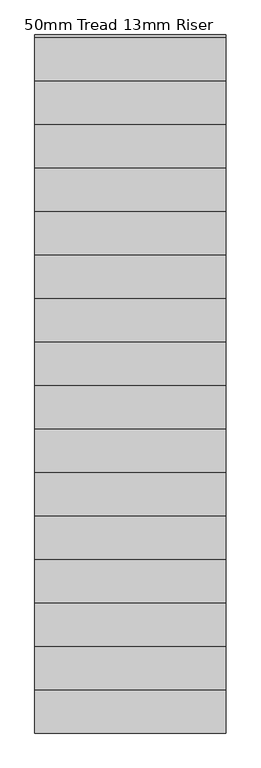
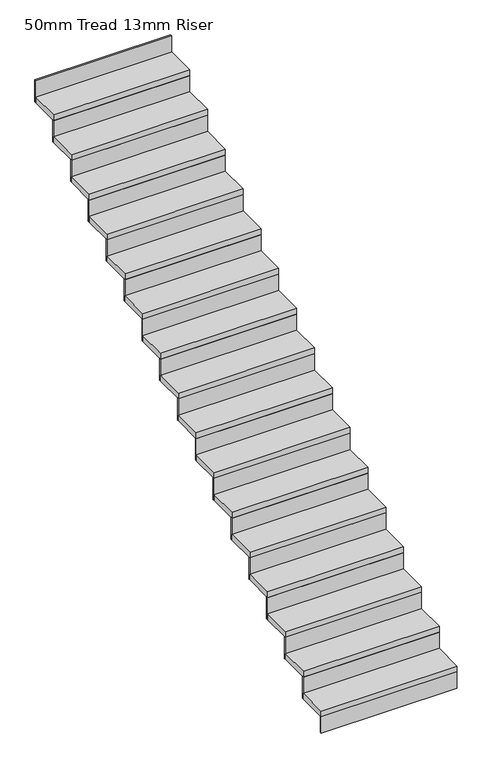
"""IFC4 building model written with IfcOpenShell, lengths in millimetres: stair flight geometry, 50mm Tread 13mm Riser."""

from ifc_helpers import new_model, si_unit, frame, origin, origin_with_axes, place, context, project, spatial, polyline, outline, extrude, source, transform, mapped, element, save


def stair_flight_50mm_tread_13mm_riser_fc77365a(model_context):
    return source(origin(), model_context, "Body", "SweptSolid", [
        extrude(outline(polyline([(-1832.0143079, -7091.702269), (-1832.0143079, -7104.202269), (-2932.0143079, -7104.202269), (-2932.0143079, -7091.702269), (-1832.0143079, -7091.702269)])), origin_with_axes(), (0.0, 0.0, 1.0), 138.2352941),
        extrude(outline(polyline([(-2932.0143079, -6854.202269), (-1832.0143079, -6854.202269), (-1832.0143079, -7104.202269), (-2932.0143079, -7104.202269), (-2932.0143079, -6854.202269)])), frame((0.0, 0.0, 138.2352941), z_axis=(0.0, 0.0, 1.0), x_axis=(1.0, 0.0, 0.0)), (0.0, 0.0, 1.0), 50.0),
        extrude(outline(polyline([(-1832.0143079, -6841.702269), (-1832.0143079, -6854.202269), (-2932.0143079, -6854.202269), (-2932.0143079, -6841.702269), (-1832.0143079, -6841.702269)])), frame((0.0, 0.0, 138.2352941), z_axis=(0.0, 0.0, 1.0), x_axis=(1.0, 0.0, 0.0)), (0.0, 0.0, 1.0), 188.2352941),
        extrude(outline(polyline([(-2932.0143079, -6604.202269), (-1832.0143079, -6604.202269), (-1832.0143079, -6854.202269), (-2932.0143079, -6854.202269), (-2932.0143079, -6604.202269)])), frame((0.0, 0.0, 326.4705882), z_axis=(0.0, 0.0, 1.0), x_axis=(1.0, 0.0, 0.0)), (0.0, 0.0, 1.0), 50.0),
        extrude(outline(polyline([(-1832.0143079, -6591.702269), (-1832.0143079, -6604.202269), (-2932.0143079, -6604.202269), (-2932.0143079, -6591.702269), (-1832.0143079, -6591.702269)])), frame((0.0, 0.0, 326.4705882), z_axis=(0.0, 0.0, 1.0), x_axis=(1.0, 0.0, 0.0)), (0.0, 0.0, 1.0), 188.2352941),
        extrude(outline(polyline([(-2932.0143079, -6354.202269), (-1832.0143079, -6354.202269), (-1832.0143079, -6604.202269), (-2932.0143079, -6604.202269), (-2932.0143079, -6354.202269)])), frame((0.0, 0.0, 514.7058824), z_axis=(0.0, 0.0, 1.0), x_axis=(1.0, 0.0, 0.0)), (0.0, 0.0, 1.0), 50.0),
        extrude(outline(polyline([(-1832.0143079, -6341.702269), (-1832.0143079, -6354.202269), (-2932.0143079, -6354.202269), (-2932.0143079, -6341.702269), (-1832.0143079, -6341.702269)])), frame((0.0, 0.0, 514.7058824), z_axis=(0.0, 0.0, 1.0), x_axis=(1.0, 0.0, 0.0)), (0.0, 0.0, 1.0), 188.2352941),
        extrude(outline(polyline([(-2932.0143079, -6104.202269), (-1832.0143079, -6104.202269), (-1832.0143079, -6354.202269), (-2932.0143079, -6354.202269), (-2932.0143079, -6104.202269)])), frame((0.0, 0.0, 702.9411765), z_axis=(0.0, 0.0, 1.0), x_axis=(1.0, 0.0, 0.0)), (0.0, 0.0, 1.0), 50.0),
        extrude(outline(polyline([(-1832.0143079, -6091.702269), (-1832.0143079, -6104.202269), (-2932.0143079, -6104.202269), (-2932.0143079, -6091.702269), (-1832.0143079, -6091.702269)])), frame((0.0, 0.0, 702.9411765), z_axis=(0.0, 0.0, 1.0), x_axis=(1.0, 0.0, 0.0)), (0.0, 0.0, 1.0), 188.2352941),
        extrude(outline(polyline([(-2932.0143079, -5854.202269), (-1832.0143079, -5854.202269), (-1832.0143079, -6104.202269), (-2932.0143079, -6104.202269), (-2932.0143079, -5854.202269)])), frame((0.0, 0.0, 891.1764706), z_axis=(0.0, 0.0, 1.0), x_axis=(1.0, 0.0, 0.0)), (0.0, 0.0, 1.0), 50.0),
        extrude(outline(polyline([(-1832.0143079, -5841.702269), (-1832.0143079, -5854.202269), (-2932.0143079, -5854.202269), (-2932.0143079, -5841.702269), (-1832.0143079, -5841.702269)])), frame((0.0, 0.0, 891.1764706), z_axis=(0.0, 0.0, 1.0), x_axis=(1.0, 0.0, 0.0)), (0.0, 0.0, 1.0), 188.2352941),
        extrude(outline(polyline([(-2932.0143079, -5604.202269), (-1832.0143079, -5604.202269), (-1832.0143079, -5854.202269), (-2932.0143079, -5854.202269), (-2932.0143079, -5604.202269)])), frame((0.0, 0.0, 1079.4117647), z_axis=(0.0, 0.0, 1.0), x_axis=(1.0, 0.0, 0.0)), (0.0, 0.0, 1.0), 50.0),
        extrude(outline(polyline([(-1832.0143079, -5591.702269), (-1832.0143079, -5604.202269), (-2932.0143079, -5604.202269), (-2932.0143079, -5591.702269), (-1832.0143079, -5591.702269)])), frame((0.0, 0.0, 1079.4117647), z_axis=(0.0, 0.0, 1.0), x_axis=(1.0, 0.0, 0.0)), (0.0, 0.0, 1.0), 188.2352941),
        extrude(outline(polyline([(-2932.0143079, -5354.202269), (-1832.0143079, -5354.202269), (-1832.0143079, -5604.202269), (-2932.0143079, -5604.202269), (-2932.0143079, -5354.202269)])), frame((0.0, 0.0, 1267.6470588), z_axis=(0.0, 0.0, 1.0), x_axis=(1.0, 0.0, 0.0)), (0.0, 0.0, 1.0), 50.0),
        extrude(outline(polyline([(-1832.0143079, -5341.702269), (-1832.0143079, -5354.202269), (-2932.0143079, -5354.202269), (-2932.0143079, -5341.702269), (-1832.0143079, -5341.702269)])), frame((0.0, 0.0, 1267.6470588), z_axis=(0.0, 0.0, 1.0), x_axis=(1.0, 0.0, 0.0)), (0.0, 0.0, 1.0), 188.2352941),
        extrude(outline(polyline([(-2932.0143079, -5104.202269), (-1832.0143079, -5104.202269), (-1832.0143079, -5354.202269), (-2932.0143079, -5354.202269), (-2932.0143079, -5104.202269)])), frame((0.0, 0.0, 1455.8823529), z_axis=(0.0, 0.0, 1.0), x_axis=(1.0, 0.0, 0.0)), (0.0, 0.0, 1.0), 50.0),
        extrude(outline(polyline([(-1832.0143079, -5091.702269), (-1832.0143079, -5104.202269), (-2932.0143079, -5104.202269), (-2932.0143079, -5091.702269), (-1832.0143079, -5091.702269)])), frame((0.0, 0.0, 1455.8823529), z_axis=(0.0, 0.0, 1.0), x_axis=(1.0, 0.0, 0.0)), (0.0, 0.0, 1.0), 188.2352941),
        extrude(outline(polyline([(-2932.0143079, -4854.202269), (-1832.0143079, -4854.202269), (-1832.0143079, -5104.202269), (-2932.0143079, -5104.202269), (-2932.0143079, -4854.202269)])), frame((0.0, 0.0, 1644.1176471), z_axis=(0.0, 0.0, 1.0), x_axis=(1.0, 0.0, 0.0)), (0.0, 0.0, 1.0), 50.0),
        extrude(outline(polyline([(-1832.0143079, -4841.702269), (-1832.0143079, -4854.202269), (-2932.0143079, -4854.202269), (-2932.0143079, -4841.702269), (-1832.0143079, -4841.702269)])), frame((0.0, 0.0, 1644.1176471), z_axis=(0.0, 0.0, 1.0), x_axis=(1.0, 0.0, 0.0)), (0.0, 0.0, 1.0), 188.2352941),
        extrude(outline(polyline([(-2932.0143079, -4604.202269), (-1832.0143079, -4604.202269), (-1832.0143079, -4854.202269), (-2932.0143079, -4854.202269), (-2932.0143079, -4604.202269)])), frame((0.0, 0.0, 1832.3529412), z_axis=(0.0, 0.0, 1.0), x_axis=(1.0, 0.0, 0.0)), (0.0, 0.0, 1.0), 50.0),
        extrude(outline(polyline([(-1832.0143079, -4591.702269), (-1832.0143079, -4604.202269), (-2932.0143079, -4604.202269), (-2932.0143079, -4591.702269), (-1832.0143079, -4591.702269)])), frame((0.0, 0.0, 1832.3529412), z_axis=(0.0, 0.0, 1.0), x_axis=(1.0, 0.0, 0.0)), (0.0, 0.0, 1.0), 188.2352941),
        extrude(outline(polyline([(-2932.0143079, -4354.202269), (-1832.0143079, -4354.202269), (-1832.0143079, -4604.202269), (-2932.0143079, -4604.202269), (-2932.0143079, -4354.202269)])), frame((0.0, 0.0, 2020.5882353), z_axis=(0.0, 0.0, 1.0), x_axis=(1.0, 0.0, 0.0)), (0.0, 0.0, 1.0), 50.0),
        extrude(outline(polyline([(-1832.0143079, -4341.702269), (-1832.0143079, -4354.202269), (-2932.0143079, -4354.202269), (-2932.0143079, -4341.702269), (-1832.0143079, -4341.702269)])), frame((0.0, 0.0, 2020.5882353), z_axis=(0.0, 0.0, 1.0), x_axis=(1.0, 0.0, 0.0)), (0.0, 0.0, 1.0), 188.2352941),
        extrude(outline(polyline([(-2932.0143079, -4104.202269), (-1832.0143079, -4104.202269), (-1832.0143079, -4354.202269), (-2932.0143079, -4354.202269), (-2932.0143079, -4104.202269)])), frame((0.0, 0.0, 2208.8235294), z_axis=(0.0, 0.0, 1.0), x_axis=(1.0, 0.0, 0.0)), (0.0, 0.0, 1.0), 50.0),
        extrude(outline(polyline([(-1832.0143079, -4091.702269), (-1832.0143079, -4104.202269), (-2932.0143079, -4104.202269), (-2932.0143079, -4091.702269), (-1832.0143079, -4091.702269)])), frame((0.0, 0.0, 2208.8235294), z_axis=(0.0, 0.0, 1.0), x_axis=(1.0, 0.0, 0.0)), (0.0, 0.0, 1.0), 188.2352941),
        extrude(outline(polyline([(-2932.0143079, -3854.202269), (-1832.0143079, -3854.202269), (-1832.0143079, -4104.202269), (-2932.0143079, -4104.202269), (-2932.0143079, -3854.202269)])), frame((0.0, 0.0, 2397.0588235), z_axis=(0.0, 0.0, 1.0), x_axis=(1.0, 0.0, 0.0)), (0.0, 0.0, 1.0), 50.0),
        extrude(outline(polyline([(-1832.0143079, -3841.702269), (-1832.0143079, -3854.202269), (-2932.0143079, -3854.202269), (-2932.0143079, -3841.702269), (-1832.0143079, -3841.702269)])), frame((0.0, 0.0, 2397.0588235), z_axis=(0.0, 0.0, 1.0), x_axis=(1.0, 0.0, 0.0)), (0.0, 0.0, 1.0), 188.2352941),
        extrude(outline(polyline([(-2932.0143079, -3604.202269), (-1832.0143079, -3604.202269), (-1832.0143079, -3854.202269), (-2932.0143079, -3854.202269), (-2932.0143079, -3604.202269)])), frame((0.0, 0.0, 2585.2941176), z_axis=(0.0, 0.0, 1.0), x_axis=(1.0, 0.0, 0.0)), (0.0, 0.0, 1.0), 50.0),
        extrude(outline(polyline([(-1832.0143079, -3591.702269), (-1832.0143079, -3604.202269), (-2932.0143079, -3604.202269), (-2932.0143079, -3591.702269), (-1832.0143079, -3591.702269)])), frame((0.0, 0.0, 2585.2941176), z_axis=(0.0, 0.0, 1.0), x_axis=(1.0, 0.0, 0.0)), (0.0, 0.0, 1.0), 188.2352941),
        extrude(outline(polyline([(-2932.0143079, -3354.202269), (-1832.0143079, -3354.202269), (-1832.0143079, -3604.202269), (-2932.0143079, -3604.202269), (-2932.0143079, -3354.202269)])), frame((0.0, 0.0, 2773.5294118), z_axis=(0.0, 0.0, 1.0), x_axis=(1.0, 0.0, 0.0)), (0.0, 0.0, 1.0), 50.0),
        extrude(outline(polyline([(-1832.0143079, -3341.702269), (-1832.0143079, -3354.202269), (-2932.0143079, -3354.202269), (-2932.0143079, -3341.702269), (-1832.0143079, -3341.702269)])), frame((0.0, 0.0, 2773.5294118), z_axis=(0.0, 0.0, 1.0), x_axis=(1.0, 0.0, 0.0)), (0.0, 0.0, 1.0), 188.2352941),
        extrude(outline(polyline([(-1832.0143079, -3091.702269), (-1832.0143079, -3104.202269), (-2932.0143079, -3104.202269), (-2932.0143079, -3091.702269), (-1832.0143079, -3091.702269)])), frame((0.0, 0.0, 2961.7647059), z_axis=(0.0, 0.0, 1.0), x_axis=(1.0, 0.0, 0.0)), (0.0, 0.0, 1.0), 188.2352941),
        extrude(outline(polyline([(-2932.0143079, -3104.202269), (-1832.0143079, -3104.202269), (-1832.0143079, -3354.202269), (-2932.0143079, -3354.202269), (-2932.0143079, -3104.202269)])), frame((0.0, 0.0, 2961.7647059), z_axis=(0.0, 0.0, 1.0), x_axis=(1.0, 0.0, 0.0)), (0.0, 0.0, 1.0), 50.0),
    ])


if __name__ == "__main__":
    model = new_model("IFC4")
    model_context = context("Model", 3, world=origin())
    ifc_project = project(units=[si_unit("LENGTHUNIT", "METRE", prefix="MILLI")], contexts=[model_context])
    site = spatial("IfcSite", under=ifc_project)
    building = spatial("IfcBuilding", under=site)
    placement = place(None, origin())
    stair_flight_50mm_tread_13mm_riser_shape = stair_flight_50mm_tread_13mm_riser_fc77365a(model_context)
    element("IfcStairFlight", 1, ObjectType="50mm Tread 13mm Riser", at=placement, inside=building, context=model_context, shape_type="MappedRepresentation", body=[
        mapped(stair_flight_50mm_tread_13mm_riser_shape, transform((0.0, 0.0, 0.0), x_axis=(1.0, 0.0, 0.0), y_axis=(0.0, 1.0, 0.0), z_axis=(0.0, 0.0, 1.0))),
    ])
    save(model, "model.ifc")

# Revit data of these elements
# Element 1 (IfcStairFlight, "50mm Tread 13mm Riser")
#   Materials on its faces: "Default"
# Materials
#   "Default": class "Generic", colour RGB 255 255 255, transparency 0, Cost = 0
